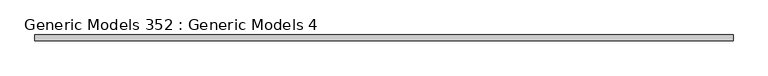
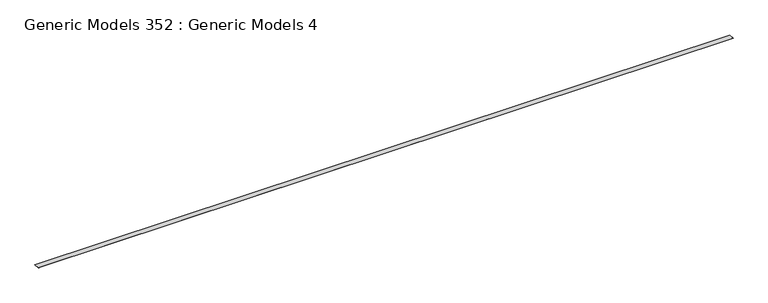
"""IFC4 building model written with IfcOpenShell, lengths in millimetres: proxy geometry, Generic Models 352 : Generic Models 4."""

from ifc_helpers import new_model, si_unit, frame, origin, place, context, project, spatial, polyline, outline, extrude, source, transform, mapped, element, save


def generic_models_352_generic_models_4_5b90fcfb(model_context):
    return source(origin(), model_context, "Body", "SweptSolid", [
        extrude(outline(polyline([(7208.2911024, 126936.7579031), (7208.2745695, 126935.9643253), (7055.1304145, 126939.1548285), (7055.1304145, 126939.9487507), (7208.2911024, 126936.7579031)])), frame((-10234.5171316, 0.0, 0.0), z_axis=(1.0, 0.0, 0.0), x_axis=(0.0, 1.0, 0.0)), (0.0, 0.0, 1.0), 18643.6),
    ])


if __name__ == "__main__":
    model = new_model("IFC4")
    model_context = context("Model", 3, world=origin())
    ifc_project = project(units=[si_unit("LENGTHUNIT", "METRE", prefix="MILLI")], contexts=[model_context])
    site = spatial("IfcSite", under=ifc_project)
    building = spatial("IfcBuilding", under=site)
    placement = place(None, origin())
    generic_models_352_generic_models_4_shape = generic_models_352_generic_models_4_5b90fcfb(model_context)
    element("IfcBuildingElementProxy", 1, Name="Generic Models 352 : Generic Models 4", ObjectType="Generic Models 352 : Generic Models 4", at=placement, inside=building, context=model_context, shape_type="MappedRepresentation", body=[
        mapped(generic_models_352_generic_models_4_shape, transform((0.0, 0.0, 0.0), x_axis=(1.0, 0.0, 0.0), y_axis=(0.0, 1.0, 0.0), z_axis=(0.0, 0.0, 1.0))),
    ])
    save(model, "model.ifc")

# Revit data of these elements
# Element 1 (IfcBuildingElementProxy, "Generic Models 352 : Generic Models 4")
#   Materials on its faces: "6\" x 4\" L FLASHING"
# Materials
#   "6\" x 4\" L FLASHING": class "Generic", colour RGB 128 0 64, transparency 0, Cost = 0
